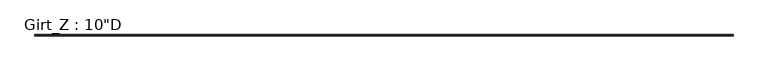
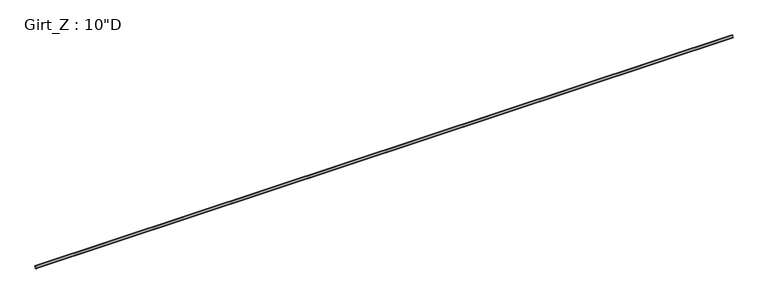
"""IFC4 building model written with IfcOpenShell, lengths in millimetres: beam geometry."""

from ifc_helpers import new_model, si_unit, point, frame, frame_2d, origin, place, context, project, spatial, polyline, circle_curve, trimmed, segment, composite_curve, outline, extrude, source, transform, mapped, element, save


def beam_2a24e19f(model_context):
    return source(origin(), model_context, "Body", "SweptSolid", [
        extrude(outline(composite_curve([segment(polyline([(63.5, 127.0), (75.745104, 112.4068534), (73.6169367, 110.621109), (62.204539, 124.221875), (3.3005807, 124.221875)]), True, "CONTINUOUS"), segment(trimmed(circle_curve(frame_2d((3.3741066, 122.2381931)), 1.9850441), [point((3.3005807, 124.221875))], [point((1.3890625, 122.2381931))], True, "CARTESIAN"), True, "CONTINUOUS"), segment(polyline([(1.3890625, 122.2381931), (1.3890625, -122.2375)]), True, "CONTINUOUS"), segment(trimmed(circle_curve(frame_2d((-3.3734375, -122.2375)), 4.7625), [point((1.3890625, -122.2375))], [point((-3.3734375, -127.0))], False, "CARTESIAN"), True, "CONTINUOUS"), segment(polyline([(-3.3734375, -127.0), (-63.5, -127.0), (-75.745104, -112.4068534), (-73.6169367, -110.621109), (-62.204539, -124.221875), (-3.2694106, -124.221875)]), True, "CONTINUOUS"), segment(trimmed(circle_curve(frame_2d((-3.3748024, -122.2389339)), 1.9857399), [point((-3.2694106, -124.221875))], [point((-1.3890625, -122.2389339))], True, "CARTESIAN"), True, "CONTINUOUS"), segment(polyline([(-1.3890625, -122.2389339), (-1.3890625, 122.2375)]), True, "CONTINUOUS"), segment(trimmed(circle_curve(frame_2d((3.3734375, 122.2375)), 4.7625), [point((-1.3890625, 122.2375))], [point((3.3734375, 127.0))], False, "CARTESIAN"), True, "CONTINUOUS"), segment(polyline([(3.3734375, 127.0), (63.5, 127.0)]), True, "CONTINUOUS")], self_intersect=False)), frame((-40373.3, 0.0, 0.0), z_axis=(1.0, 0.0, 0.0), x_axis=(0.0, 1.0, 0.0)), (0.0, 0.0, 1.0), 80505.2999999),
    ])


if __name__ == "__main__":
    model = new_model("IFC4")
    model_context = context("Model", 3, world=origin())
    ifc_project = project(units=[si_unit("LENGTHUNIT", "METRE", prefix="MILLI")], contexts=[model_context])
    site = spatial("IfcSite", under=ifc_project)
    building = spatial("IfcBuilding", under=site)
    placement = place(None, origin())
    beam_shape = beam_2a24e19f(model_context)
    element("IfcBeam", 1, ObjectType="Girt_Z : 10\"D", at=placement, inside=building, context=model_context, shape_type="MappedRepresentation", body=[
        mapped(beam_shape, transform((0.0, 0.0, 0.0), x_axis=(1.0, 0.0, 0.0), y_axis=(0.0, 1.0, 0.0), z_axis=(0.0, 0.0, 1.0))),
    ])
    save(model, "model.ifc")

# Revit data of these elements
# Type "Girt_Z : 10\"D"
#   Web_Thickness = 0' - 0 7/64"
#   Length [instance default] = 10' - 0"
#   Leg_1 = 0' - 2 1/2"
#   Height = 0' - 10"
#   Structural Material [instance default] = none
# Element 1 (IfcBeam, "Girt_Z : 10\"D")
#   Structural Material = Steel
#   Materials on its faces: "Steel"
# Materials
#   "Steel": class "Metal", colour RGB 118 118 114, transparency 0, Description = "Steel, mill finish", Cost = 0
